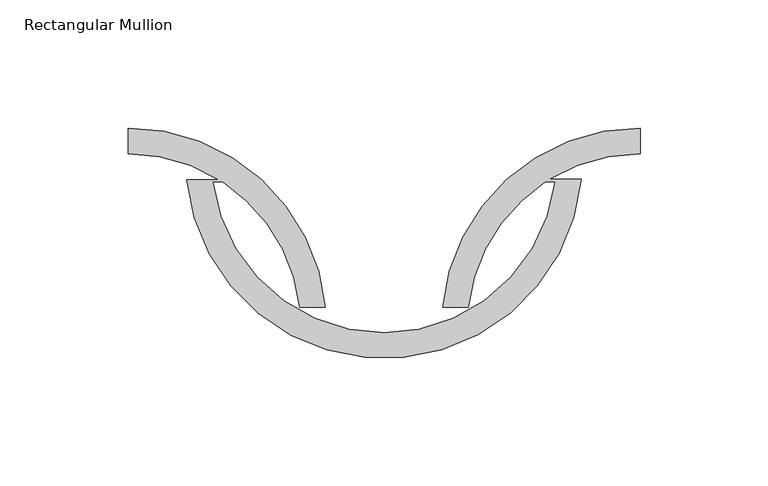
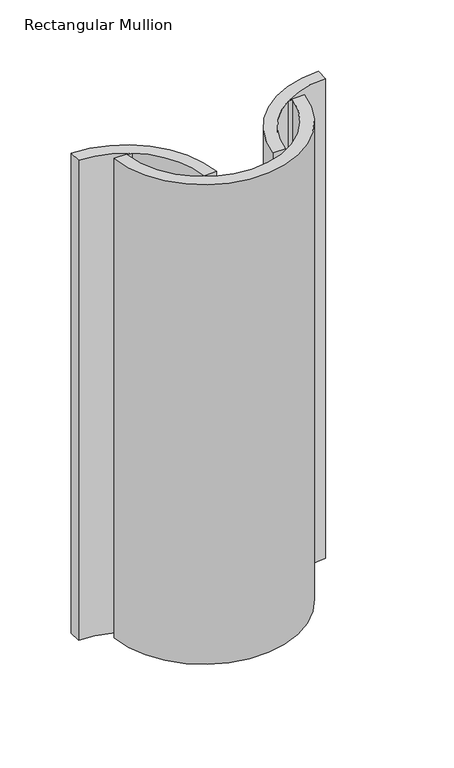
"""IFC4 building model written with IfcOpenShell, lengths in millimetres: member geometry, Rectangular Mullion : Telha Cerâmica - Colonial."""

from ifc_helpers import new_model, si_unit, point, frame, frame_2d, origin, place, context, project, spatial, polyline, circle_curve, trimmed, segment, composite_curve, outline, extrude, source, transform, mapped, element, save


def rectangular_mullion_79a2ef4b(model_context):
    return source(origin(), model_context, "Body", "SweptSolid", [
        extrude(outline(composite_curve([segment(polyline([(-77.1836628, -20.1172602), (-64.5135712, -20.1172602)]), True, "CONTINUOUS"), segment(trimmed(circle_curve(frame_2d((-100.058911, -77.5)), 67.5), [point((-64.5135712, -20.1172602))], [point((-100.058911, -10.0))], True, "CARTESIAN"), True, "CONTINUOUS"), segment(polyline([(-100.058911, -10.0), (-100.058911, 0.0)]), True, "CONTINUOUS"), segment(trimmed(circle_curve(frame_2d((-100.058911, -77.5)), 77.5), [point((-100.058911, 0.0))], [point((-22.9226679, -70.0))], False, "CARTESIAN"), True, "CONTINUOUS"), segment(polyline([(-22.9226679, -70.0), (-32.9768716, -70.0)]), True, "CONTINUOUS"), segment(trimmed(circle_curve(frame_2d((-100.058911, -77.5)), 67.5), [point((-32.9768716, -70.0))], [point((-63.1265403, -21.0))], True, "CARTESIAN"), True, "CONTINUOUS"), segment(polyline([(-63.1265403, -21.0), (-67.0215871, -21.0)]), True, "CONTINUOUS"), segment(trimmed(circle_curve(frame_2d((-0.058911, -12.5)), 67.5), [point((-67.0215871, -21.0))], [point((66.9037652, -21.0))], True, "CARTESIAN"), True, "CONTINUOUS"), segment(polyline([(66.9037652, -21.0), (63.0087184, -21.0)]), True, "CONTINUOUS"), segment(trimmed(circle_curve(frame_2d((99.941089, -77.5)), 67.5), [point((63.0087184, -21.0))], [point((32.8590497, -70.0))], True, "CARTESIAN"), True, "CONTINUOUS"), segment(polyline([(32.8590497, -70.0), (22.8048459, -70.0)]), True, "CONTINUOUS"), segment(trimmed(circle_curve(frame_2d((99.941089, -77.5)), 77.5), [point((22.8048459, -70.0))], [point((99.941089, 0.0))], False, "CARTESIAN"), True, "CONTINUOUS"), segment(polyline([(99.941089, 0.0), (99.941089, -10.0)]), True, "CONTINUOUS"), segment(trimmed(circle_curve(frame_2d((99.941089, -77.5)), 67.5), [point((99.941089, -10.0))], [point((64.58575, -20.0))], True, "CARTESIAN"), True, "CONTINUOUS"), segment(polyline([(64.58575, -20.0), (77.0773321, -20.0)]), True, "CONTINUOUS"), segment(trimmed(circle_curve(frame_2d((-0.058911, -12.5)), 77.5), [point((77.0773321, -20.0))], [point((-77.1836628, -20.1172602))], False, "CARTESIAN"), True, "CONTINUOUS")], self_intersect=False)), frame((0.0, 0.0, -410.0), z_axis=(0.0, 0.0, 1.0), x_axis=(1.0, 0.0, 0.0)), (0.0, 0.0, 1.0), 410.0),
    ])


if __name__ == "__main__":
    model = new_model("IFC4")
    model_context = context("Model", 3, world=origin())
    ifc_project = project(units=[si_unit("LENGTHUNIT", "METRE", prefix="MILLI")], contexts=[model_context])
    site = spatial("IfcSite", under=ifc_project)
    building = spatial("IfcBuilding", under=site)
    placement = place(None, origin())
    rectangular_mullion_shape = rectangular_mullion_79a2ef4b(model_context)
    element("IfcMember", 1, ObjectType="Rectangular Mullion : Telha Cerâmica - Colonial", at=placement, inside=building, context=model_context, shape_type="MappedRepresentation", body=[
        mapped(rectangular_mullion_shape, transform((0.0, 0.0, 0.0), x_axis=(1.0, 0.0, 0.0), y_axis=(0.0, 1.0, 0.0), z_axis=(0.0, 0.0, 1.0))),
    ])
    save(model, "model.ifc")

# Revit data of these elements
# Type "Rectangular Mullion : Telha Cerâmica - Colonial"
#   built-in parameter 1007322 = 0.0328084 (stored number, unit not read)
#   built-in parameter 1007321 = 0.327891 (stored number, unit not read)
#   built-in parameter 1007320 = 0.328277 (stored number, unit not read)
# Element 1 (IfcMember, "Rectangular Mullion : Telha Cerâmica - Colonial")
#   Materials on its faces: "Telha - Cerâmica"
# Materials
#   "Telha - Cerâmica": class "Cerâmica", colour RGB 68 35 31, transparency 0, Description = "Interior finish", Cost = 0
